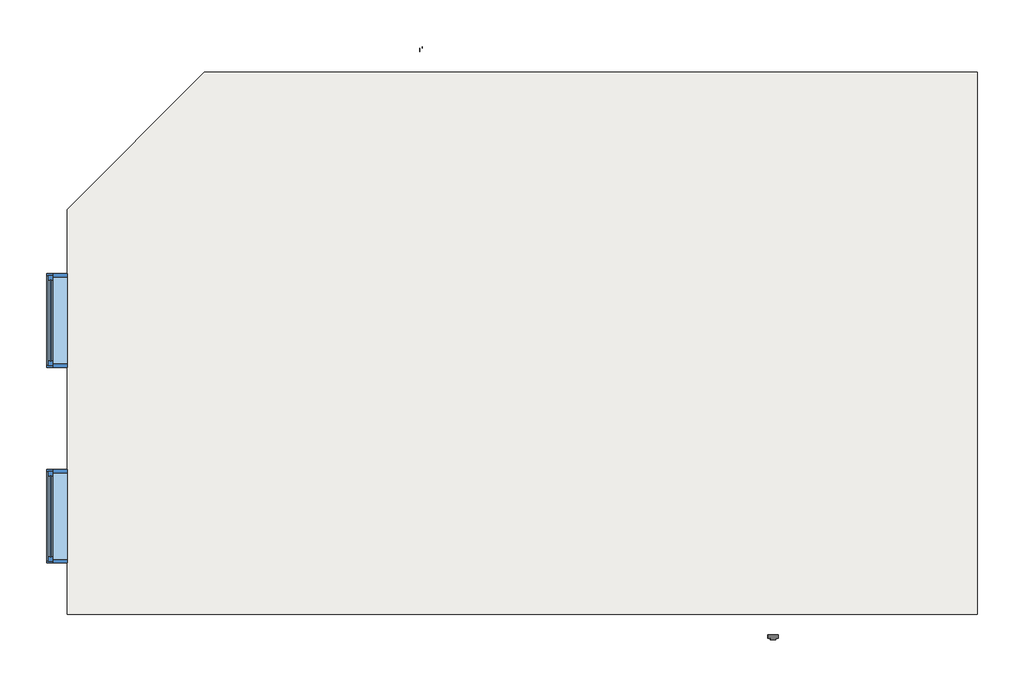
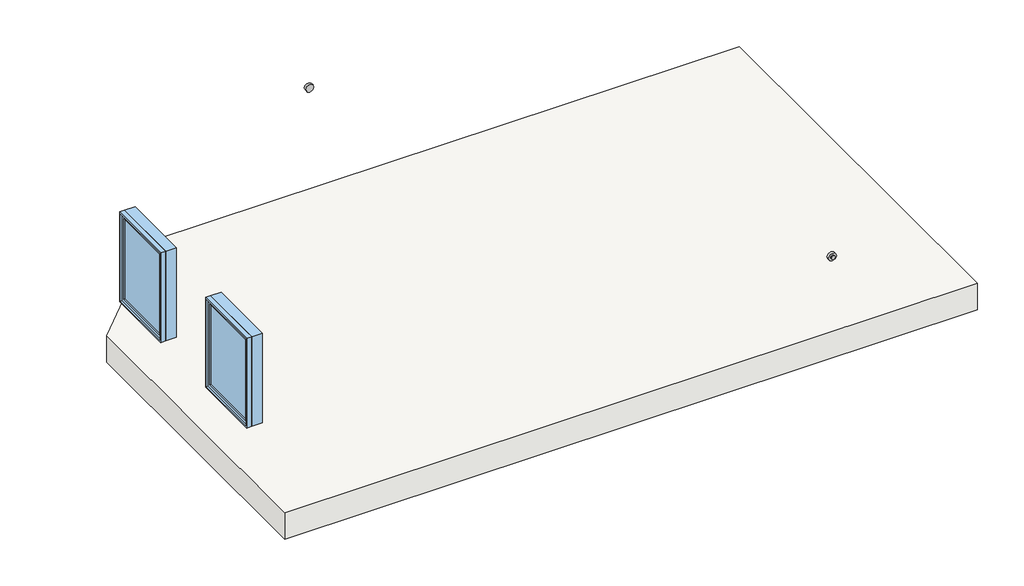
# One storey: 2 alarms, 2 windows, 1 slab.
"""IFC4 building model written with IfcOpenShell, lengths in millimetres."""

import ifcopenshell
import ifcopenshell.guid

model = None  # the IFC model being written
_history = None  # IfcOwnerHistory: only IFC2X3 demands one
_inside = {}  # id of a spatial element -> (the spatial element, [elements in it])
_under = {}  # id of a project, library or spatial element -> (it, [spatial elements below it])
_declared = {}  # id of a project -> (the project, [libraries it declares])
_typed = {}  # id of a type object -> (the type object, [elements of that type])
_made_of = {}  # id of a material, layer set ... -> (it, [elements and type objects made of it])


def new_model(schema):
    """Start an empty IFC model of exactly this schema.

    Asked for "IFC4X3", IfcOpenShell would pick the latest addendum, in which some entities
    have other attributes; the version numbers below select the first issue.
    IFC2X3 requires an IfcOwnerHistory on every rooted entity: one is made here for all.
    """
    global model, _history
    if schema == "IFC4X3":
        model = ifcopenshell.file(schema_version=(4, 3, 0, 0))
    else:
        model = ifcopenshell.file(schema=schema)
    _inside.clear()
    _under.clear()
    _declared.clear()
    _typed.clear()
    _made_of.clear()
    _history = None
    if model.schema == "IFC2X3":
        org = make("IfcOrganization", Name="unknown")
        user = make(
            "IfcPersonAndOrganization",
            ThePerson=make("IfcPerson", FamilyName="unknown"),
            TheOrganization=org,
        )
        app = make(
            "IfcApplication",
            ApplicationDeveloper=org,
            Version="unknown",
            ApplicationFullName="unknown",
            ApplicationIdentifier="unknown",
        )
        _history = make(
            "IfcOwnerHistory",
            OwningUser=user,
            OwningApplication=app,
            ChangeAction="ADDED",
            CreationDate=0,
        )
    return model


def make(cls, **values):
    """One entity of the class cls with the attributes given. An attribute that is None is left unset."""
    return model.create_entity(
        cls, **{name: value for name, value in values.items() if value is not None}
    )


def rooted(cls, **values):
    """An entity with a GlobalId (a new one), such as an element, a storey or a relation."""
    return make(cls, GlobalId=ifcopenshell.guid.new(), OwnerHistory=_history, **values)


def si_unit(unit_type, name, prefix=None):
    """IfcSIUnit, for example si_unit("LENGTHUNIT", "METRE", prefix="MILLI")."""
    return make("IfcSIUnit", UnitType=unit_type, Prefix=prefix, Name=name)


def assignment(units):
    """IfcUnitAssignment: the units of a project."""
    return None if units is None else make("IfcUnitAssignment", Units=units)


def point(xyz):
    """IfcCartesianPoint."""
    return None if xyz is None else make("IfcCartesianPoint", Coordinates=xyz)


def direction(xyz):
    """IfcDirection."""
    return None if xyz is None else make("IfcDirection", DirectionRatios=xyz)


def frame(location, z_axis=None, x_axis=None):
    """IfcAxis2Placement3D, a coordinate frame: its origin and axes. An axis left out is left unset."""
    return make(
        "IfcAxis2Placement3D",
        Location=point(location),
        Axis=direction(z_axis),
        RefDirection=direction(x_axis),
    )


def origin():
    """The frame at (0, 0, 0) with its axes left unset."""
    return frame((0.0, 0.0, 0.0))


def origin_with_axes():
    """The frame at (0, 0, 0) with the z axis (0, 0, 1) and the x axis (1, 0, 0) written out."""
    return frame((0.0, 0.0, 0.0), z_axis=(0.0, 0.0, 1.0), x_axis=(1.0, 0.0, 0.0))


def place(relative_to, where):
    """IfcLocalPlacement: puts the frame where relative to a parent placement (None: the world)."""
    return make(
        "IfcLocalPlacement", PlacementRelTo=relative_to, RelativePlacement=where
    )


def context(
    kind, dimensions, precision=None, world=None, true_north=None, identifier=None
):
    """IfcGeometricRepresentationContext, for example the 3D "Model" context."""
    return make(
        "IfcGeometricRepresentationContext",
        ContextIdentifier=identifier,
        ContextType=kind,
        CoordinateSpaceDimension=dimensions,
        Precision=precision,
        WorldCoordinateSystem=world,
        TrueNorth=true_north,
    )


def project(units=None, contexts=None):
    """IfcProject with its units and contexts."""
    return rooted(
        "IfcProject",
        Name="project",
        RepresentationContexts=contexts,
        UnitsInContext=assignment(units),
    )


def spatial(cls, under=None, at=None, **own):
    """A site, building, storey or space (cls), placed at a placement, below another one or the project."""
    s = rooted(cls, ObjectPlacement=at, **own)
    if under is not None:
        _under.setdefault(under.id(), (under, []))[1].append(s)
    return s


def polyline(points):
    """IfcPolyline through the points."""
    return make("IfcPolyline", Points=[point(p) for p in points])


def circle_curve(where, radius):
    """IfcCircle in the frame where."""
    return make("IfcCircle", Position=where, Radius=radius)


def outline(outer, holes=None, kind="AREA"):
    """IfcArbitraryClosedProfileDef: a profile drawn as a closed curve; with holes, ...WithVoids."""
    if holes is None:
        return make("IfcArbitraryClosedProfileDef", ProfileType=kind, OuterCurve=outer)
    return make(
        "IfcArbitraryProfileDefWithVoids",
        ProfileType=kind,
        OuterCurve=outer,
        InnerCurves=holes,
    )


def extrude(swept, where, along, depth):
    """IfcExtrudedAreaSolid: the profile swept, set in the frame where, extruded along a direction by depth."""
    return make(
        "IfcExtrudedAreaSolid",
        SweptArea=swept,
        Position=where,
        ExtrudedDirection=direction(along),
        Depth=depth,
    )


def shape(context_of_items, identifier, shape_type, items):
    """IfcShapeRepresentation: the items that make up one representation, for example the "Body"."""
    return make(
        "IfcShapeRepresentation",
        ContextOfItems=context_of_items,
        RepresentationIdentifier=identifier,
        RepresentationType=shape_type,
        Items=items,
    )


def source(mapping_origin, context_of_items, identifier, shape_type, items):
    """IfcRepresentationMap: a shape defined once, which mapped items show again and again."""
    return make(
        "IfcRepresentationMap",
        MappingOrigin=mapping_origin,
        MappedRepresentation=shape(context_of_items, identifier, shape_type, items),
    )


def transform(
    local_origin,
    x_axis=None,
    y_axis=None,
    z_axis=None,
    scale=None,
    scale2=None,
    scale3=None,
    uniform=True,
):
    """IfcCartesianTransformationOperator3D, or its non-uniform kind. x_axis, y_axis, z_axis: its Axis1, 2, 3."""
    if uniform:
        return make(
            "IfcCartesianTransformationOperator3D",
            Axis1=direction(x_axis),
            Axis2=direction(y_axis),
            LocalOrigin=point(local_origin),
            Scale=scale,
            Axis3=direction(z_axis),
        )
    return make(
        "IfcCartesianTransformationOperator3DnonUniform",
        Axis1=direction(x_axis),
        Axis2=direction(y_axis),
        LocalOrigin=point(local_origin),
        Scale=scale,
        Axis3=direction(z_axis),
        Scale2=scale2,
        Scale3=scale3,
    )


def mapped(mapping_source, mapping_target):
    """IfcMappedItem: shows the shape of a source again, moved by a transform."""
    return make(
        "IfcMappedItem", MappingSource=mapping_source, MappingTarget=mapping_target
    )


def made_of(thing, what):
    """Note that an element or type object is made of a material, layer set ...; save() writes the relation."""
    if what is not None:
        _made_of.setdefault(what.id(), (what, []))[1].append(thing)
    return thing


def element(
    cls,
    number,
    at=None,
    inside=None,
    cuts=None,
    type_object=None,
    material=None,
    context=None,
    identifier="Body",
    shape_type=None,
    held_by="IfcProductDefinitionShape",
    body=None,
    shapes=None,
    **own,
):
    """One element of the class cls, such as IfcWall. Its Tag is "e" and its number.

    at: its placement. inside: the storey or other place that contains it. cuts: it is an
    opening in that element (IfcRelVoidsElement). A single representation is given by context,
    identifier, shape_type and body (its items); several are given by shapes. held_by: the class
    of the entity that holds the representations. save() writes the other relations.
    """
    e = rooted(cls, Tag="e%d" % number, ObjectPlacement=at, **own)
    if body is not None:
        shapes = [shape(context, identifier, shape_type, body)]
    if shapes is not None:
        e.Representation = make(held_by, Representations=shapes)
    if inside is not None:
        _inside.setdefault(inside.id(), (inside, []))[1].append(e)
    if cuts is not None:
        rooted(
            "IfcRelVoidsElement", RelatingBuildingElement=cuts, RelatedOpeningElement=e
        )
    if type_object is not None:
        _typed.setdefault(type_object.id(), (type_object, []))[1].append(e)
    return made_of(e, material)


def aggregate(whole, parts):
    """IfcRelAggregates: a whole, such as a stair, and the parts it consists of."""
    return rooted("IfcRelAggregates", RelatingObject=whole, RelatedObjects=parts)


def save(model, path):
    """Write the relations noted so far, then the file.

    IfcRelAggregates (storeys below a building ...), IfcRelContainedInSpatialStructure (elements
    in a storey), IfcRelDefinesByType, IfcRelAssociatesMaterial and IfcRelDeclares: one each for
    every whole, place, type object, material and project.
    """
    for whole, parts in _under.values():
        aggregate(whole, parts)
    for where, things in _inside.values():
        rooted(
            "IfcRelContainedInSpatialStructure",
            RelatedElements=things,
            RelatingStructure=where,
        )
    for kind, things in _typed.values():
        rooted("IfcRelDefinesByType", RelatedObjects=things, RelatingType=kind)
    for what, things in _made_of.values():
        rooted("IfcRelAssociatesMaterial", RelatedObjects=things, RelatingMaterial=what)
    for by, libraries in _declared.values():
        rooted("IfcRelDeclares", RelatingContext=by, RelatedDefinitions=libraries)
    model.write(path)


def plane_surface(at):
    """IfcPlane: the flat surface through the origin of the frame at, square to its z axis."""
    return make("IfcPlane", Position=at)


def cylinder_surface(at, radius):
    """IfcCylindricalSurface: all points at the distance radius from the z axis of the frame at."""
    return make("IfcCylindricalSurface", Position=at, Radius=radius)


def advanced_brep(points, edges, surfaces, faces):
    """IfcAdvancedBrep: a solid bounded by faces that lie on surfaces and meet in shared edges.

    An edge is (start, end): straight between two places in points (the first is 0);
    or (start, end, curve); or (start, end, curve, False) where it runs against its curve.
    A face is (place in surfaces, loops), or (place, loops, False) where it looks against
    its surface's normal. A loop lists edges by number (the first is 1), with a minus sign
    where the edge is run from its end to its start. The first loop is the outer one.
    """
    corners = [point(p) for p in points]
    vertices = [make("IfcVertexPoint", VertexGeometry=c) for c in corners]
    made = []
    for start, end, *more in edges:
        made.append(
            make(
                "IfcEdgeCurve",
                EdgeStart=vertices[start],
                EdgeEnd=vertices[end],
                EdgeGeometry=more[0] if more else make("IfcPolyline", Points=[corners[start], corners[end]]),
                SameSense=more[1] if len(more) > 1 else True,
            )
        )
    hull = []
    for where, loops, *sense in faces:
        bounds = []
        for j, loop in enumerate(loops):
            ring = [make("IfcOrientedEdge", EdgeElement=made[abs(k) - 1], Orientation=k > 0) for k in loop]
            bounds.append(
                make(
                    "IfcFaceOuterBound" if j == 0 else "IfcFaceBound",
                    Bound=make("IfcEdgeLoop", EdgeList=ring),
                    Orientation=True,
                )
            )
        hull.append(make("IfcAdvancedFace", Bounds=bounds, FaceSurface=surfaces[where], SameSense=sense[0] if sense else True))
    return make("IfcAdvancedBrep", Outer=make("IfcClosedShell", CfsFaces=hull))


def alarm_5285ee31(model_context):
    return source(origin(), model_context, "Body", "AdvancedBrep", [
        advanced_brep(
        [(-26.0, 0.0, 50.0), (26.0, 0.0, 50.0), (-52.0, 0.0, 0.0), (52.0, 0.0, 0.0), (-26.0, 0.0, 35.0), (26.0, 0.0, 35.0), (-52.0, 0.0, 35.0), (52.0, 0.0, 35.0)],
        [
            (0, 1, circle_curve(frame((0.0, 0.0, 50.0), z_axis=(0.0, 0.0, 1.0), x_axis=(1.0, 0.0, 0.0)), 26.0)),
            (1, 0, circle_curve(frame((0.0, 0.0, 50.0), z_axis=(0.0, 0.0, 1.0), x_axis=(1.0, 0.0, 0.0)), 26.0)),
            (2, 3, circle_curve(frame((0.0, 0.0, 0.0), z_axis=(0.0, 0.0, -1.0), x_axis=(1.0, 0.0, 0.0)), 52.0)),
            (3, 2, circle_curve(frame((0.0, 0.0, 0.0), z_axis=(0.0, 0.0, -1.0), x_axis=(1.0, 0.0, 0.0)), 52.0)),
            (0, 4),
            (4, 5, circle_curve(frame((0.0, 0.0, 35.0), z_axis=(0.0, 0.0, 1.0), x_axis=(1.0, 0.0, 0.0)), 26.0)),
            (5, 1),
            (5, 4, circle_curve(frame((0.0, 0.0, 35.0), z_axis=(0.0, 0.0, 1.0), x_axis=(1.0, 0.0, 0.0)), 26.0)),
            (6, 7, circle_curve(frame((0.0, 0.0, 35.0), z_axis=(0.0, 0.0, 1.0), x_axis=(1.0, 0.0, 0.0)), 52.0)),
            (7, 6, circle_curve(frame((0.0, 0.0, 35.0), z_axis=(0.0, 0.0, 1.0), x_axis=(1.0, 0.0, 0.0)), 52.0)),
            (3, 7),
            (6, 2),
        ],
        [
            plane_surface(frame((26.0, 0.0, 50.0), z_axis=(0.0, 0.0, 1.0), x_axis=(0.0, 1.0, 0.0))),
            plane_surface(frame((26.0, 0.0, 0.0), z_axis=(0.0, 0.0, -1.0), x_axis=(0.0, -1.0, 0.0))),
            cylinder_surface(origin_with_axes(), 26.0),
            plane_surface(frame((52.0, 0.0, 35.0), z_axis=(0.0, 0.0, 1.0), x_axis=(0.0, 1.0, 0.0))),
            cylinder_surface(origin_with_axes(), 52.0),
        ],
        [
            (0, [[1, 2]]),
            (1, [[3, 4]]),
            (2, [[-1, 5, 6, 7]]),
            (2, [[-2, -7, 8, -5]]),
            (3, [[9, 10], [-6, -8]]),
            (4, [[-4, 11, -9, 12]]),
            (4, [[-3, -12, -10, -11]]),
        ],
    ),
    ])


def window_0915_x_1220mm_488fb2fb(model_context):
    return source(origin(), model_context, "Body", "SweptSolid", [
        extrude(outline(polyline([(-394.5, 78.0), (394.5, 78.0), (394.5, 66.0), (-394.5, 66.0), (-394.5, 78.0)])), frame((0.0, 0.0, 978.0), z_axis=(0.0, 0.0, 1.0), x_axis=(1.0, 0.0, 0.0)), (0.0, 0.0, 1.0), 1094.0),
        extrude(outline(polyline([(2116.0, -438.5), (934.0, -438.5), (934.0, 438.5), (2116.0, 438.5), (2116.0, -438.5)]), holes=[polyline([(2072.0, -394.5), (2072.0, 394.5), (978.0, 394.5), (978.0, -394.5), (2072.0, -394.5)])]), frame((0.0, 50.0, 0.0), z_axis=(0.0, 1.0, 0.0), x_axis=(0.0, 0.0, 1.0)), (0.0, 0.0, 1.0), 44.0),
        extrude(outline(polyline([(2135.0, -457.5), (915.0, -457.5), (915.0, 457.5), (2135.0, 457.5), (2135.0, -457.5)]), holes=[polyline([(2116.0, -438.5), (2116.0, 438.5), (934.0, 438.5), (934.0, -438.5), (2116.0, -438.5)])]), frame((0.0, 50.0, 0.0), z_axis=(0.0, 1.0, 0.0), x_axis=(0.0, 0.0, 1.0)), (0.0, 0.0, 1.0), 63.0),
        extrude(outline(polyline([(2135.0, -457.5), (915.0, -457.5), (915.0, 457.5), (2135.0, 457.5), (2135.0, -457.5)]), holes=[polyline([(2103.0, -425.5), (2103.0, 425.5), (947.0, 425.5), (947.0, -425.5), (2103.0, -425.5)])]), frame((0.0, -87.0, 0.0), z_axis=(0.0, 1.0, 0.0), x_axis=(0.0, 0.0, 1.0)), (0.0, 0.0, 1.0), 137.0),
    ])


model = new_model("IFC4")

# Units and contexts
model_context = context("Model", 3, world=origin())
ifc_project = project(units=[si_unit("LENGTHUNIT", "METRE", prefix="MILLI")], contexts=[model_context])

# Site, building, storey
site = spatial("IfcSite", under=ifc_project)
building = spatial("IfcBuilding", under=site)
storey = spatial("IfcBuildingStorey", under=building, Name="标高 2", Elevation=4000.0)

# Alarms
placement = place(None, origin())
alarm_shape = alarm_5285ee31(model_context)
element("IfcAlarm", 1, ObjectType="光电感烟探测器 : 点型", at=placement, inside=storey, context=model_context, shape_type="MappedRepresentation", body=[
    mapped(alarm_shape, transform((-580.1449608, -867.5409421, 5200.0), x_axis=(1.0, 0.0, 0.0), y_axis=(0.0, 0.0, 1.0), z_axis=(0.0, -1.0, 0.0))),
])
element("IfcAlarm", 2, ObjectType="光电感烟探测器 : 点型", at=placement, inside=storey, context=model_context, shape_type="MappedRepresentation", body=[
    mapped(alarm_shape, transform((-3980.1449608, 4838.4590579, 5200.0), x_axis=(0.9993908270190954, 0.0, 0.03489949670251135), y_axis=(0.03489949670251135, 0.0, -0.9993908270190954), z_axis=(0.0, 1.0, 0.0))),
])

# Slab
element("IfcSlab", 3, ObjectType="混凝土 - 商用 362mm", at=placement, inside=storey, context=model_context, shape_type="SweptSolid", body=[
    extrude(outline(polyline([(-6138.7236046, 4635.4590579), (1419.8550392, 4635.4590579), (1419.8550392, -664.5409421), (-7480.1449608, -664.5409421), (-7480.1449608, 3294.0377016), (-6138.7236046, 4635.4590579)])), frame((0.0, 0.0, 3638.0), z_axis=(0.0, 0.0, 1.0), x_axis=(1.0, 0.0, 0.0)), (0.0, 0.0, 1.0), 362.0),
])

# Windows
window_0915_x_1220mm_shape = window_0915_x_1220mm_488fb2fb(model_context)
element("IfcWindow", 4, ObjectType="固定 : 0915 x 1220mm", at=placement, inside=storey, context=model_context, shape_type="MappedRepresentation", body=[
    mapped(window_0915_x_1220mm_shape, transform((-7567.1449608, 292.9590579, 4000.0), x_axis=(0.0, 1.0, 0.0), y_axis=(-1.0, 0.0, 0.0), z_axis=(0.0, 0.0, 1.0))),
])
element("IfcWindow", 5, ObjectType="固定 : 0915 x 1220mm", at=placement, inside=storey, context=model_context, shape_type="MappedRepresentation", body=[
    mapped(window_0915_x_1220mm_shape, transform((-7567.1449608, 2207.9590579, 4000.0), x_axis=(0.0, 1.0, 0.0), y_axis=(-1.0, 0.0, 0.0), z_axis=(0.0, 0.0, 1.0))),
])

save(model, "model.ifc")

# Revit data of these elements
# Type "光电感烟探测器 : 点型"
#   半径 3 = 36.77 mm
#   半径 2 = 52 mm
#   半径 1 = 26 mm
#   高度 2 = 15 mm
#   高度 1 = 35 mm
#   Default Elevation = 1200 mm
#   可见性 2 = no
#   可见性 1 = yes
#   材质 = none
# Type "混凝土 - 商用 362mm"
#   Function = 0
#   Layers, outside or top first: 200 mm "混凝土 - 现场浇注" (function 1); 0 mm "防湿" (function 100); 12 mm "沙" (function 0); 150 mm "场地 - 碎石" (function 0)
# Type "固定 : 0915 x 1220mm"
#   Type Mark = "15"
#   Construction Type Id = "GSP4R"
#   Analytic Construction = "1/8 英寸 Pilkington 单层玻璃"
#   Visual Light Transmittance = 0.9
#   Solar Heat Gain Coefficient = 0.78
#   Heat Transfer Coefficient (U) = 3.6886 W/(m²·K)
#   Height = 1220 mm
#   默认窗台高度 = 915 mm
#   Width = 915 mm
#   窗嵌入 = 19 mm
#   框架外部材质 = 窗扇
#   框架内部材质 = 窗扇
#   玻璃嵌板材质 = 玻璃
#   窗扇 = 窗扇
#   Wall Closure = (empty or 0)
# Element 1 (IfcAlarm, "光电感烟探测器 : 点型")
#   Comments = "光电传感器-22..."
#   Mark = "2"
#   Phase Created = 阶段 1
# Element 2 (IfcAlarm, "光电感烟探测器 : 点型")
#   Mark = "3"
#   Phase Created = 阶段 1
# Element 3 (IfcSlab, "混凝土 - 商用 362mm")
#   built-in parameter 1001955 = 0.785398 (stored number, unit not read)
#   Height Offset From Level = 0 mm
#   Phase Created = 阶段 1
#   Materials on its faces: "场地 - 碎石", "混凝土 - 现场浇注"
# Element 4 (IfcWindow, "固定 : 0915 x 1220mm")
#   Mark = "6"
#   Phase Created = 阶段 1
#   Materials on its faces: "窗扇", "玻璃"
# Element 5 (IfcWindow, "固定 : 0915 x 1220mm")
#   Mark = "7"
#   Phase Created = 阶段 1
#   Materials on its faces: "窗扇", "玻璃"
# Materials
#   "混凝土 - 现场浇注": class "混凝土", colour RGB 192 192 192, transparency 0, Cost = 0
#   "防湿": class "常规", colour RGB 127 127 127, transparency 0, Description = "防湿", Cost = 0
#   "沙": class "常规", colour RGB 191 183 178, transparency 0, Description = "沙", Cost = 0
#   "场地 - 碎石": class "其他", colour RGB 165 42 42, transparency 0, Cost = 0
#   "窗扇": class "木质", colour RGB 224 178 126, transparency 0, Cost = 0
#   "玻璃": class "玻璃", colour RGB 0 128 192, transparency 0.9, Description = "钠钙玻璃", Cost = 0
